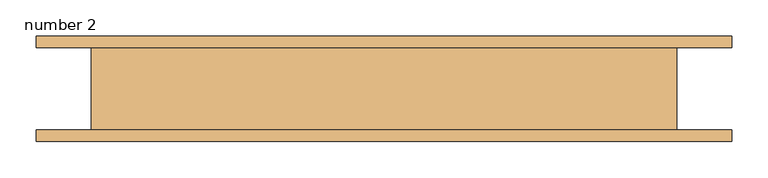
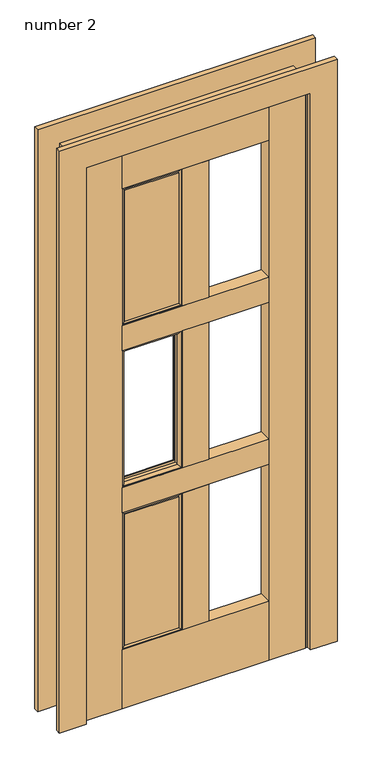
"""IFC4 building model written with IfcOpenShell, lengths in millimetres: door geometry, Door-Interior-Karona-K5660-6_Panel : number 2."""

from ifc_helpers import new_model, si_unit, frame, origin, origin_with_axes, place, context, project, spatial, polyline, ellipse_curve, outline, extrude, faceted_brep, source, transform, mapped, element, save
from ifc_brep_helpers import plane_surface, cylinder_surface, revolved_surface, advanced_brep


def number_2_d489d55d(model_context):
    return source(origin(), model_context, "Body", "SolidModel", [
        advanced_brep(
        [(-254.0, -15.2908, 1311.275), (-46.0375, -15.2908, 1311.275), (-57.3628137, -24.6126, 1299.9496863), (-242.6746863, -24.6126, 1299.9496863), (-57.1627, -46.3324899, 1300.1498), (-57.1627, -46.3324899, 820.7502), (-48.2727, -54.4576, 811.8602), (-48.2727, -54.4576, 1309.0398), (-242.8748, -46.3324899, 820.7502), (-242.8748, -46.3324899, 1300.1498), (-251.7648, -54.4576, 1309.0398), (-251.7648, -54.4576, 811.8602), (-46.0375, -54.4576, 809.625), (-254.0, -54.4576, 809.625), (-254.0, -15.2908, 809.625), (-46.0375, -15.2908, 809.625), (-57.1627, -34.7218, 820.7502), (-242.8748, -34.7218, 820.7502), (-47.3075, -24.6126, 1310.005), (-47.3075, -24.6126, 810.895), (-47.3075, -34.7218, 810.895), (-47.3075, -34.7218, 1310.005), (-252.73, -24.6126, 810.895), (-252.73, -24.6126, 1310.005), (-57.3628137, -24.6126, 820.9503137), (-242.6746863, -24.6126, 820.9503137), (-252.73, -34.7218, 810.895), (-254.0, -54.4576, 1311.275), (-242.8748, -34.7218, 1300.1498), (-252.73, -34.7218, 1310.005), (-46.0375, -54.4576, 1311.275), (-57.1627, -34.7218, 1300.1498)],
        [
            (0, 1),
            (1, 2, ellipse_curve(frame((-47.0685124, -25.5788135, 1310.2439876), z_axis=(-0.7071067811865475, 0.0, 0.7071067811865475), x_axis=(-0.7071067811865476, 0.0, -0.7071067811865474)), 14.6223259, 10.3395458)),
            (2, 3),
            (3, 0, ellipse_curve(frame((-252.9689876, -25.5788135, 1310.2439876), z_axis=(0.7071067811865475, 0.0, 0.7071067811865475), x_axis=(-0.7071067811865476, 0.0, 0.7071067811865474)), 14.6223259, 10.3395458)),
            (4, 5),
            (5, 6, ellipse_curve(frame((-48.2727, -45.531597, 811.8602), z_axis=(0.7071067811865475, 0.0, 0.7071067811865475), x_axis=(-0.7071067811865474, 0.0, 0.7071067811865476)), 12.6232745, 8.926003)),
            (6, 7),
            (7, 4, ellipse_curve(frame((-48.2727, -45.531597, 1309.0398), z_axis=(0.7071067811865475, 0.0, -0.7071067811865475), x_axis=(0.7071067811865474, 0.0, 0.7071067811865476)), 12.6232745, 8.926003)),
            (8, 9),
            (9, 10, ellipse_curve(frame((-251.7648, -45.531597, 1309.0398), z_axis=(-0.7071067811865475, 0.0, -0.7071067811865475), x_axis=(0.7071067811865474, 0.0, -0.7071067811865476)), 12.6232745, 8.926003)),
            (10, 11),
            (11, 8, ellipse_curve(frame((-251.7648, -45.531597, 811.8602), z_axis=(-0.7071067811865475, 0.0, 0.7071067811865475), x_axis=(-0.7071067811865474, 0.0, -0.7071067811865476)), 12.6232745, 8.926003)),
            (12, 13),
            (13, 14),
            (14, 15),
            (15, 12),
            (16, 17),
            (17, 8),
            (8, 5),
            (5, 16),
            (18, 19),
            (19, 20),
            (20, 21),
            (21, 18),
            (22, 19),
            (18, 23),
            (23, 22),
            (24, 25),
            (25, 3),
            (2, 24),
            (14, 25, ellipse_curve(frame((-252.9689876, -25.5788135, 810.6560124), z_axis=(0.7071067811865475, 0.0, -0.7071067811865475), x_axis=(0.7071067811865476, 0.0, 0.7071067811865474)), 14.6223259, 10.3395458)),
            (24, 15, ellipse_curve(frame((-47.0685124, -25.5788135, 810.6560124), z_axis=(-0.7071067811865475, 0.0, -0.7071067811865475), x_axis=(0.7071067811865476, 0.0, -0.7071067811865474)), 14.6223259, 10.3395458)),
            (22, 26),
            (26, 20),
            (13, 27),
            (27, 0),
            (0, 14),
            (17, 28),
            (28, 9),
            (23, 29),
            (29, 26),
            (27, 30),
            (30, 1),
            (28, 31),
            (31, 4),
            (4, 9),
            (21, 29),
            (30, 12),
            (15, 1),
            (31, 16),
            (6, 11),
            (10, 7),
        ],
        [
            cylinder_surface(frame((-254.0, -25.5788135, 1310.2439876), z_axis=(-1.0, 0.0, 0.0), x_axis=(0.0, 1.0, 0.0)), 10.3395458),
            cylinder_surface(frame((-48.2727, -45.531597, 1311.275), z_axis=(0.0, 0.0, 1.0), x_axis=(0.0, 1.0, 0.0)), 8.926003),
            cylinder_surface(frame((-251.7648, -45.531597, 809.625), z_axis=(0.0, 0.0, -1.0), x_axis=(0.0, 1.0, 0.0)), 8.926003),
            plane_surface(frame((-46.0375, -15.2908, 809.625), z_axis=(0.0, 0.0, -1.0), x_axis=(-1.0, 0.0, 0.0))),
            plane_surface(frame((-57.1627, -46.3324899, 820.7502), z_axis=(0.0, 0.0, 1.0), x_axis=(-1.0, 0.0, 0.0))),
            plane_surface(frame((-47.3075, -34.7218, 1310.005), z_axis=(-1.0, 0.0, 0.0), x_axis=(0.0, 0.0, -1.0))),
            plane_surface(frame((-47.3075, -24.6126, 1310.005), z_axis=(0.0, -1.0, 0.0), x_axis=(0.0, 0.0, -1.0))),
            cylinder_surface(frame((-46.0375, -25.5788135, 810.6560124), z_axis=(1.0, 0.0, 0.0), x_axis=(0.0, 1.0, 0.0)), 10.3395458),
            plane_surface(frame((-47.3075, -34.7218, 810.895), z_axis=(0.0, 0.0, 1.0), x_axis=(-1.0, 0.0, 0.0))),
            plane_surface(frame((-254.0, -15.2908, 809.625), z_axis=(-1.0, 0.0, 0.0), x_axis=(0.0, 0.0, 1.0))),
            plane_surface(frame((-242.8748, -46.3324899, 820.7502), z_axis=(1.0, 0.0, 0.0), x_axis=(0.0, 0.0, 1.0))),
            plane_surface(frame((-252.73, -34.7218, 810.895), z_axis=(1.0, 0.0, 0.0), x_axis=(0.0, 0.0, 1.0))),
            plane_surface(frame((-254.0, -15.2908, 1311.275), z_axis=(0.0, 0.0, 1.0), x_axis=(1.0, 0.0, 0.0))),
            plane_surface(frame((-242.8748, -46.3324899, 1300.1498), z_axis=(0.0, 0.0, -1.0), x_axis=(1.0, 0.0, 0.0))),
            plane_surface(frame((-252.73, -34.7218, 1310.005), z_axis=(0.0, 0.0, -1.0), x_axis=(1.0, 0.0, 0.0))),
            plane_surface(frame((-46.0375, -15.2908, 1311.275), z_axis=(1.0, 0.0, 0.0), x_axis=(0.0, 0.0, -1.0))),
            plane_surface(frame((-57.1627, -46.3324899, 1300.1498), z_axis=(-1.0, 0.0, 0.0), x_axis=(0.0, 0.0, -1.0))),
            plane_surface(frame((-57.1627, -34.7218, 1300.1498), z_axis=(0.0, 1.0, 0.0), x_axis=(0.0, 0.0, -1.0))),
            plane_surface(frame((-46.0375, -54.4576, 1311.275), z_axis=(0.0, -1.0, 0.0), x_axis=(0.0, 0.0, -1.0))),
            cylinder_surface(frame((-46.0375, -45.531597, 811.8602), z_axis=(1.0, 0.0, 0.0), x_axis=(0.0, 1.0, 0.0)), 8.926003),
            cylinder_surface(frame((-252.9689876, -25.5788135, 809.625), z_axis=(0.0, 0.0, -1.0), x_axis=(0.0, 1.0, 0.0)), 10.3395458),
            cylinder_surface(frame((-254.0, -45.531597, 1309.0398), z_axis=(-1.0, 0.0, 0.0), x_axis=(0.0, 1.0, 0.0)), 8.926003),
            cylinder_surface(frame((-47.0685124, -25.5788135, 1311.275), z_axis=(0.0, 0.0, 1.0), x_axis=(0.0, 1.0, 0.0)), 10.3395458),
        ],
        [
            (0, [[1, 2, 3, 4]]),
            (1, [[5, 6, 7, 8]]),
            (2, [[9, 10, 11, 12]]),
            (3, [[13, 14, 15, 16]]),
            (4, [[17, 18, 19, 20]]),
            (5, [[21, 22, 23, 24]]),
            (6, [[25, -21, 26, 27], [28, 29, -3, 30]]),
            (7, [[-15, 31, -28, 32]]),
            (8, [[-25, 33, 34, -22]]),
            (9, [[35, 36, 37, -14]]),
            (10, [[38, 39, -9, -18]]),
            (11, [[-27, 40, 41, -33]]),
            (12, [[42, 43, -1, -36]]),
            (13, [[44, 45, 46, -39]]),
            (14, [[-26, -24, 47, -40]]),
            (15, [[48, -16, 49, -43]]),
            (16, [[50, -20, -5, -45]]),
            (17, [[-34, -41, -47, -23], [-17, -50, -44, -38]]),
            (18, [[-13, -48, -42, -35], [51, -11, 52, -7]]),
            (19, [[-19, -12, -51, -6]]),
            (20, [[-37, -4, -29, -31]]),
            (21, [[-46, -8, -52, -10]]),
            (22, [[-49, -32, -30, -2]]),
        ],
    ),
        advanced_brep(
        [(-242.8748, -54.4576, 1893.8748), (-242.8748, -54.4576, 1414.4752), (-57.1627, -54.4576, 1414.4752), (-57.1627, -54.4576, 1893.8748), (-242.8748, -34.7218, 1893.8748), (-242.8748, -36.0454899, 1893.8748), (-57.1627, -36.0454899, 1893.8748), (-57.1627, -34.7218, 1893.8748), (-57.1627, -44.5515929, 1893.8748), (-242.8748, -44.5515929, 1893.8748), (-57.1627, -34.7218, 1414.4752), (-57.1627, -36.0454899, 1414.4752), (-242.8748, -36.0454899, 1414.4752), (-242.8748, -34.7218, 1414.4752), (-242.8748, -44.5515929, 1414.4752), (-57.1627, -44.5515929, 1414.4752), (-87.1686653, -44.5515929, 1863.8688347), (-212.8688347, -44.5515929, 1863.8688347), (-87.1686653, -44.5515929, 1444.4811653), (-212.8688347, -44.5515929, 1444.4811653)],
        [
            (0, 1),
            (1, 2),
            (2, 3),
            (3, 0),
            (4, 5),
            (5, 6),
            (6, 7),
            (7, 4),
            (3, 8),
            (8, 9),
            (9, 0),
            (10, 11),
            (11, 12),
            (12, 13),
            (13, 10),
            (1, 14),
            (14, 15),
            (15, 2),
            (9, 14),
            (12, 5),
            (4, 13),
            (6, 11),
            (10, 7),
            (15, 8),
            (16, 6, ellipse_curve(frame((-55.2243315, -100.0605261, 1895.8131685), z_axis=(0.7071067811865475, 0.0, -0.7071067811865475), x_axis=(-0.7071067811865476, 0.0, -0.7071067811865474)), 90.5724254, 64.0443762)),
            (5, 17, ellipse_curve(frame((-244.8131685, -100.0605261, 1895.8131685), z_axis=(-0.7071067811865475, 0.0, -0.7071067811865475), x_axis=(-0.7071067811865476, 0.0, 0.7071067811865474)), 90.5724254, 64.0443762)),
            (17, 16),
            (18, 11, ellipse_curve(frame((-55.2243315, -100.0605261, 1412.5368315), z_axis=(-0.7071067811865475, 0.0, -0.7071067811865475), x_axis=(-0.7071067811865474, 0.0, 0.7071067811865476)), 90.5724254, 64.0443762)),
            (16, 18),
            (19, 12, ellipse_curve(frame((-244.8131685, -100.0605261, 1412.5368315), z_axis=(-0.7071067811865475, 0.0, 0.7071067811865475), x_axis=(0.7071067811865476, 0.0, 0.7071067811865474)), 90.5724254, 64.0443762)),
            (18, 19),
            (19, 17),
        ],
        [
            plane_surface(frame((-57.1627, -54.4576, 1893.8748), z_axis=(0.0, -1.0, 0.0), x_axis=(0.0, 0.0, -1.0))),
            plane_surface(frame((-57.1627, -34.7218, 1893.8748), z_axis=(0.0, 0.0, 1.0), x_axis=(1.0, 0.0, 0.0))),
            plane_surface(frame((-57.1627, -34.7218, 1414.4752), z_axis=(0.0, 0.0, -1.0), x_axis=(-1.0, 0.0, 0.0))),
            plane_surface(frame((-242.8748, -54.4576, 1893.8748), z_axis=(-1.0, 0.0, 0.0), x_axis=(0.0, 0.0, -1.0))),
            plane_surface(frame((-57.1627, -34.7218, 1893.8748), z_axis=(1.0, 0.0, 0.0), x_axis=(0.0, 0.0, -1.0))),
            plane_surface(frame((-242.8748, -34.7218, 1893.8748), z_axis=(0.0, 1.0, 0.0), x_axis=(0.0, 0.0, -1.0))),
            revolved_surface(polyline([(-308.8575446888527, -100.0605261, 1831.7687923), (8.820044688852704, -100.0605261, 1831.7687923)]), (-254.0, -100.0605261, 1895.8131685), (-1.0, 0.0, 0.0)),
            revolved_surface(polyline([(-119.2687077, -100.0605261, 1959.8575446888528), (-119.2687077, -100.0605261, 1348.4924553111473)]), (-55.2243315, -100.0605261, 1905.0), (0.0, 0.0, 1.0)),
            revolved_surface(polyline([(8.820044688852683, -100.0605261, 1476.5812077), (-308.8575446888527, -100.0605261, 1476.5812077)]), (-46.0375, -100.0605261, 1412.5368315), (1.0, 0.0, 0.0)),
            revolved_surface(polyline([(-180.76879229999997, -100.0605261, 1348.4924553111473), (-180.76879229999997, -100.0605261, 1959.8575446888526)]), (-244.8131685, -100.0605261, 1403.35), (0.0, 0.0, -1.0)),
            plane_surface(frame((-254.0, -44.5515929, 1403.35), z_axis=(0.0, 1.0, 0.0), x_axis=(0.0, 0.0, 1.0))),
        ],
        [
            (0, [[1, 2, 3, 4]]),
            (1, [[5, 6, 7, 8]]),
            (1, [[9, 10, 11, -4]]),
            (2, [[12, 13, 14, 15]]),
            (2, [[16, 17, 18, -2]]),
            (3, [[-11, 19, -16, -1]]),
            (3, [[-14, 20, -5, 21]]),
            (4, [[-7, 22, -12, 23]]),
            (4, [[-18, 24, -9, -3]]),
            (5, [[-23, -15, -21, -8]]),
            (6, [[25, -6, 26, 27]]),
            (7, [[28, -22, -25, 29]]),
            (8, [[30, -13, -28, 31]]),
            (9, [[-26, -20, -30, 32]]),
            (10, [[-24, -17, -19, -10], [-32, -31, -29, -27]]),
        ],
    ),
        advanced_brep(
        [(-242.8748, -24.6126, 1893.8748), (-242.8748, -24.6126, 1414.4752), (-57.1627, -24.6126, 1414.4752), (-57.1627, -24.6126, 1893.8748), (-214.0448579, -15.4432, 1443.3051421), (-214.0448579, -15.4432, 1865.0448579), (-85.9926421, -15.4432, 1865.0448579), (-85.9926421, -15.4432, 1443.3051421), (-57.1627, -23.2889101, 1893.8748), (-242.8748, -23.2889101, 1893.8748), (-242.8748, -23.2889101, 1414.4752), (-57.1627, -23.2889101, 1414.4752)],
        [
            (0, 1),
            (1, 2),
            (2, 3),
            (3, 0),
            (4, 5),
            (5, 6),
            (6, 7),
            (7, 4),
            (3, 8),
            (8, 9),
            (9, 0),
            (1, 10),
            (10, 11),
            (11, 2),
            (7, 11, ellipse_curve(frame((-55.2243315, 40.7261261, 1412.5368315), z_axis=(0.7071067811865475, 0.0, 0.7071067811865475), x_axis=(0.7071067811865476, 0.0, -0.7071067811865474)), 90.5724254, 64.0443762)),
            (10, 4, ellipse_curve(frame((-244.8131685, 40.7261261, 1412.5368315), z_axis=(-0.7071067811865475, 0.0, 0.7071067811865475), x_axis=(0.7071067811865476, 0.0, 0.7071067811865474)), 90.5724254, 64.0443762)),
            (10, 9),
            (9, 5, ellipse_curve(frame((-244.8131685, 40.7261261, 1895.8131685), z_axis=(0.7071067811865475, 0.0, 0.7071067811865475), x_axis=(0.7071067811865474, 0.0, -0.7071067811865476)), 90.5724254, 64.0443762)),
            (8, 6, ellipse_curve(frame((-55.2243315, 40.7261261, 1895.8131685), z_axis=(0.7071067811865475, 0.0, -0.7071067811865475), x_axis=(-0.7071067811865476, 0.0, -0.7071067811865474)), 90.5724254, 64.0443762)),
            (8, 11),
        ],
        [
            plane_surface(frame((-57.1627, -24.6126, 1893.8748), z_axis=(0.0, -1.0, 0.0), x_axis=(0.0, 0.0, -1.0))),
            plane_surface(frame((-242.8748, -15.4432, 1893.8748), z_axis=(0.0, 1.0, 0.0), x_axis=(0.0, 0.0, -1.0))),
            plane_surface(frame((-57.1627, -34.7218, 1893.8748), z_axis=(0.0, 0.0, 1.0), x_axis=(1.0, 0.0, 0.0))),
            plane_surface(frame((-57.1627, -34.7218, 1414.4752), z_axis=(0.0, 0.0, -1.0), x_axis=(-1.0, 0.0, 0.0))),
            revolved_surface(polyline([(8.820044688852711, 40.7261261, 1476.5812077), (-308.8575446888527, 40.7261261, 1476.5812077)]), (-46.0375, 40.7261261, 1412.5368315), (1.0, 0.0, 0.0)),
            revolved_surface(polyline([(-180.76879229999997, 40.7261261, 1348.4924553111473), (-180.76879229999997, 40.7261261, 1959.8575446888528)]), (-244.8131685, 40.7261261, 1403.35), (0.0, 0.0, -1.0)),
            revolved_surface(polyline([(-308.85754468885267, 40.7261261, 1831.7687923), (8.820044688852704, 40.7261261, 1831.7687923)]), (-254.0, 40.7261261, 1895.8131685), (-1.0, 0.0, 0.0)),
            revolved_surface(polyline([(-119.2687077, 40.7261261, 1959.8575446888528), (-119.2687077, 40.7261261, 1348.4924553111473)]), (-55.2243315, 40.7261261, 1905.0), (0.0, 0.0, 1.0)),
            plane_surface(frame((-242.8748, -24.6126, 1893.8748), z_axis=(-1.0, 0.0, 0.0), x_axis=(0.0, 0.0, -1.0))),
            plane_surface(frame((-57.1627, -15.4432, 1893.8748), z_axis=(1.0, 0.0, 0.0), x_axis=(0.0, 0.0, -1.0))),
        ],
        [
            (0, [[1, 2, 3, 4]]),
            (1, [[5, 6, 7, 8]]),
            (2, [[9, 10, 11, -4]]),
            (3, [[12, 13, 14, -2]]),
            (4, [[-8, 15, -13, 16]]),
            (5, [[17, 18, -5, -16]]),
            (6, [[-10, 19, -6, -18]]),
            (7, [[20, -15, -7, -19]]),
            (8, [[-11, -17, -12, -1]]),
            (9, [[-14, -20, -9, -3]]),
        ],
    ),
        advanced_brep(
        [(-254.0, -15.2908, 1905.0), (-46.0375, -15.2908, 1905.0), (-57.3628137, -24.6126, 1893.6746863), (-242.6746863, -24.6126, 1893.6746863), (-57.1627, -46.3324899, 1893.8748), (-57.1627, -46.3324899, 1414.4752), (-48.2727, -54.4576, 1405.5852), (-48.2727, -54.4576, 1902.7648), (-242.8748, -46.3324899, 1414.4752), (-242.8748, -46.3324899, 1893.8748), (-251.7648, -54.4576, 1902.7648), (-251.7648, -54.4576, 1405.5852), (-46.0375, -54.4576, 1403.35), (-254.0, -54.4576, 1403.35), (-254.0, -15.2908, 1403.35), (-46.0375, -15.2908, 1403.35), (-57.1627, -34.7218, 1414.4752), (-242.8748, -34.7218, 1414.4752), (-47.3075, -24.6126, 1903.73), (-47.3075, -24.6126, 1404.62), (-47.3075, -34.7218, 1404.62), (-47.3075, -34.7218, 1903.73), (-252.73, -24.6126, 1404.62), (-252.73, -24.6126, 1903.73), (-57.3628137, -24.6126, 1414.6753137), (-242.6746863, -24.6126, 1414.6753137), (-252.73, -34.7218, 1404.62), (-254.0, -54.4576, 1905.0), (-242.8748, -34.7218, 1893.8748), (-252.73, -34.7218, 1903.73), (-46.0375, -54.4576, 1905.0), (-57.1627, -34.7218, 1893.8748)],
        [
            (0, 1),
            (1, 2, ellipse_curve(frame((-47.0685124, -25.5788135, 1903.9689876), z_axis=(-0.7071067811865475, 0.0, 0.7071067811865475), x_axis=(-0.7071067811865476, 0.0, -0.7071067811865474)), 14.6223259, 10.3395458)),
            (2, 3),
            (3, 0, ellipse_curve(frame((-252.9689876, -25.5788135, 1903.9689876), z_axis=(0.7071067811865475, 0.0, 0.7071067811865475), x_axis=(-0.7071067811865476, 0.0, 0.7071067811865474)), 14.6223259, 10.3395458)),
            (4, 5),
            (5, 6, ellipse_curve(frame((-48.2727, -45.531597, 1405.5852), z_axis=(0.7071067811865475, 0.0, 0.7071067811865475), x_axis=(-0.7071067811865474, 0.0, 0.7071067811865476)), 12.6232745, 8.926003)),
            (6, 7),
            (7, 4, ellipse_curve(frame((-48.2727, -45.531597, 1902.7648), z_axis=(0.7071067811865475, 0.0, -0.7071067811865475), x_axis=(0.7071067811865474, 0.0, 0.7071067811865476)), 12.6232745, 8.926003)),
            (8, 9),
            (9, 10, ellipse_curve(frame((-251.7648, -45.531597, 1902.7648), z_axis=(-0.7071067811865475, 0.0, -0.7071067811865475), x_axis=(0.7071067811865474, 0.0, -0.7071067811865476)), 12.6232745, 8.926003)),
            (10, 11),
            (11, 8, ellipse_curve(frame((-251.7648, -45.531597, 1405.5852), z_axis=(-0.7071067811865475, 0.0, 0.7071067811865475), x_axis=(-0.7071067811865474, 0.0, -0.7071067811865476)), 12.6232745, 8.926003)),
            (12, 13),
            (13, 14),
            (14, 15),
            (15, 12),
            (16, 17),
            (17, 8),
            (8, 5),
            (5, 16),
            (18, 19),
            (19, 20),
            (20, 21),
            (21, 18),
            (22, 19),
            (18, 23),
            (23, 22),
            (24, 25),
            (25, 3),
            (2, 24),
            (14, 25, ellipse_curve(frame((-252.9689876, -25.5788135, 1404.3810124), z_axis=(0.7071067811865475, 0.0, -0.7071067811865475), x_axis=(0.7071067811865476, 0.0, 0.7071067811865474)), 14.6223259, 10.3395458)),
            (24, 15, ellipse_curve(frame((-47.0685124, -25.5788135, 1404.3810124), z_axis=(-0.7071067811865475, 0.0, -0.7071067811865475), x_axis=(0.7071067811865476, 0.0, -0.7071067811865474)), 14.6223259, 10.3395458)),
            (22, 26),
            (26, 20),
            (13, 27),
            (27, 0),
            (0, 14),
            (17, 28),
            (28, 9),
            (23, 29),
            (29, 26),
            (27, 30),
            (30, 1),
            (28, 31),
            (31, 4),
            (4, 9),
            (21, 29),
            (30, 12),
            (15, 1),
            (31, 16),
            (6, 11),
            (10, 7),
        ],
        [
            cylinder_surface(frame((-254.0, -25.5788135, 1903.9689876), z_axis=(-1.0, 0.0, 0.0), x_axis=(0.0, 1.0, 0.0)), 10.3395458),
            cylinder_surface(frame((-48.2727, -45.531597, 1905.0), z_axis=(0.0, 0.0, 1.0), x_axis=(0.0, 1.0, 0.0)), 8.926003),
            cylinder_surface(frame((-251.7648, -45.531597, 1403.35), z_axis=(0.0, 0.0, -1.0), x_axis=(0.0, 1.0, 0.0)), 8.926003),
            plane_surface(frame((-46.0375, -15.2908, 1403.35), z_axis=(0.0, 0.0, -1.0), x_axis=(-1.0, 0.0, 0.0))),
            plane_surface(frame((-57.1627, -46.3324899, 1414.4752), z_axis=(0.0, 0.0, 1.0), x_axis=(-1.0, 0.0, 0.0))),
            plane_surface(frame((-47.3075, -34.7218, 1903.73), z_axis=(-1.0, 0.0, 0.0), x_axis=(0.0, 0.0, -1.0))),
            plane_surface(frame((-47.3075, -24.6126, 1903.73), z_axis=(0.0, -1.0, 0.0), x_axis=(0.0, 0.0, -1.0))),
            cylinder_surface(frame((-46.0375, -25.5788135, 1404.3810124), z_axis=(1.0, 0.0, 0.0), x_axis=(0.0, 1.0, 0.0)), 10.3395458),
            plane_surface(frame((-47.3075, -34.7218, 1404.62), z_axis=(0.0, 0.0, 1.0), x_axis=(-1.0, 0.0, 0.0))),
            plane_surface(frame((-254.0, -15.2908, 1403.35), z_axis=(-1.0, 0.0, 0.0), x_axis=(0.0, 0.0, 1.0))),
            plane_surface(frame((-242.8748, -46.3324899, 1414.4752), z_axis=(1.0, 0.0, 0.0), x_axis=(0.0, 0.0, 1.0))),
            plane_surface(frame((-252.73, -34.7218, 1404.62), z_axis=(1.0, 0.0, 0.0), x_axis=(0.0, 0.0, 1.0))),
            plane_surface(frame((-254.0, -15.2908, 1905.0), z_axis=(0.0, 0.0, 1.0), x_axis=(1.0, 0.0, 0.0))),
            plane_surface(frame((-242.8748, -46.3324899, 1893.8748), z_axis=(0.0, 0.0, -1.0), x_axis=(1.0, 0.0, 0.0))),
            plane_surface(frame((-252.73, -34.7218, 1903.73), z_axis=(0.0, 0.0, -1.0), x_axis=(1.0, 0.0, 0.0))),
            plane_surface(frame((-46.0375, -15.2908, 1905.0), z_axis=(1.0, 0.0, 0.0), x_axis=(0.0, 0.0, -1.0))),
            plane_surface(frame((-57.1627, -46.3324899, 1893.8748), z_axis=(-1.0, 0.0, 0.0), x_axis=(0.0, 0.0, -1.0))),
            plane_surface(frame((-57.1627, -34.7218, 1893.8748), z_axis=(0.0, 1.0, 0.0), x_axis=(0.0, 0.0, -1.0))),
            plane_surface(frame((-46.0375, -54.4576, 1905.0), z_axis=(0.0, -1.0, 0.0), x_axis=(0.0, 0.0, -1.0))),
            cylinder_surface(frame((-46.0375, -45.531597, 1405.5852), z_axis=(1.0, 0.0, 0.0), x_axis=(0.0, 1.0, 0.0)), 8.926003),
            cylinder_surface(frame((-252.9689876, -25.5788135, 1403.35), z_axis=(0.0, 0.0, -1.0), x_axis=(0.0, 1.0, 0.0)), 10.3395458),
            cylinder_surface(frame((-254.0, -45.531597, 1902.7648), z_axis=(-1.0, 0.0, 0.0), x_axis=(0.0, 1.0, 0.0)), 8.926003),
            cylinder_surface(frame((-47.0685124, -25.5788135, 1905.0), z_axis=(0.0, 0.0, 1.0), x_axis=(0.0, 1.0, 0.0)), 10.3395458),
        ],
        [
            (0, [[1, 2, 3, 4]]),
            (1, [[5, 6, 7, 8]]),
            (2, [[9, 10, 11, 12]]),
            (3, [[13, 14, 15, 16]]),
            (4, [[17, 18, 19, 20]]),
            (5, [[21, 22, 23, 24]]),
            (6, [[25, -21, 26, 27], [28, 29, -3, 30]]),
            (7, [[-15, 31, -28, 32]]),
            (8, [[-25, 33, 34, -22]]),
            (9, [[35, 36, 37, -14]]),
            (10, [[38, 39, -9, -18]]),
            (11, [[-27, 40, 41, -33]]),
            (12, [[42, 43, -1, -36]]),
            (13, [[44, 45, 46, -39]]),
            (14, [[-26, -24, 47, -40]]),
            (15, [[48, -16, 49, -43]]),
            (16, [[50, -20, -5, -45]]),
            (17, [[-34, -41, -47, -23], [-17, -50, -44, -38]]),
            (18, [[-13, -48, -42, -35], [51, -11, 52, -7]]),
            (19, [[-19, -12, -51, -6]]),
            (20, [[-37, -4, -29, -31]]),
            (21, [[-46, -8, -52, -10]]),
            (22, [[-49, -32, -30, -2]]),
        ],
    ),
        advanced_brep(
        [(-242.8748, -34.7218, 706.4248), (-242.8748, -36.0454899, 706.4248), (-57.1627, -36.0454899, 706.4248), (-57.1627, -34.7218, 706.4248), (-57.1627, -54.4576, 706.4248), (-57.1627, -44.5515929, 706.4248), (-242.8748, -44.5515929, 706.4248), (-242.8748, -54.4576, 706.4248), (-57.1627, -34.7218, 227.0252), (-57.1627, -36.0454899, 227.0252), (-242.8748, -36.0454899, 227.0252), (-242.8748, -34.7218, 227.0252), (-242.8748, -54.4576, 227.0252), (-242.8748, -44.5515929, 227.0252), (-57.1627, -44.5515929, 227.0252), (-57.1627, -54.4576, 227.0252), (-87.1686653, -44.5515929, 676.4188347), (-212.8688347, -44.5515929, 676.4188347), (-87.1686653, -44.5515929, 257.0311653), (-212.8688347, -44.5515929, 257.0311653)],
        [
            (0, 1),
            (1, 2),
            (2, 3),
            (3, 0),
            (4, 5),
            (5, 6),
            (6, 7),
            (7, 4),
            (8, 9),
            (9, 10),
            (10, 11),
            (11, 8),
            (12, 13),
            (13, 14),
            (14, 15),
            (15, 12),
            (6, 13),
            (12, 7),
            (10, 1),
            (0, 11),
            (15, 4),
            (2, 9),
            (8, 3),
            (14, 5),
            (16, 2, ellipse_curve(frame((-55.2243315, -100.0605261, 708.3631685), z_axis=(0.7071067811865475, 0.0, -0.7071067811865475), x_axis=(-0.7071067811865476, 0.0, -0.7071067811865474)), 90.5724254, 64.0443762)),
            (1, 17, ellipse_curve(frame((-244.8131685, -100.0605261, 708.3631685), z_axis=(-0.7071067811865475, 0.0, -0.7071067811865475), x_axis=(-0.7071067811865476, 0.0, 0.7071067811865474)), 90.5724254, 64.0443762)),
            (17, 16),
            (18, 9, ellipse_curve(frame((-55.2243315, -100.0605261, 225.0868315), z_axis=(-0.7071067811865475, 0.0, -0.7071067811865475), x_axis=(-0.7071067811865474, 0.0, 0.7071067811865476)), 90.5724254, 64.0443762)),
            (16, 18),
            (19, 10, ellipse_curve(frame((-244.8131685, -100.0605261, 225.0868315), z_axis=(-0.7071067811865475, 0.0, 0.7071067811865475), x_axis=(0.7071067811865476, 0.0, 0.7071067811865474)), 90.5724254, 64.0443762)),
            (18, 19),
            (19, 17),
        ],
        [
            plane_surface(frame((-57.1627, -34.7218, 706.4248), z_axis=(0.0, 0.0, 1.0), x_axis=(1.0, 0.0, 0.0))),
            plane_surface(frame((-57.1627, -34.7218, 227.0252), z_axis=(0.0, 0.0, -1.0), x_axis=(-1.0, 0.0, 0.0))),
            plane_surface(frame((-242.8748, -54.4576, 706.4248), z_axis=(-1.0, 0.0, 0.0), x_axis=(0.0, 0.0, -1.0))),
            plane_surface(frame((-57.1627, -54.4576, 706.4248), z_axis=(0.0, -1.0, 0.0), x_axis=(0.0, 0.0, -1.0))),
            plane_surface(frame((-57.1627, -34.7218, 706.4248), z_axis=(1.0, 0.0, 0.0), x_axis=(0.0, 0.0, -1.0))),
            plane_surface(frame((-242.8748, -34.7218, 706.4248), z_axis=(0.0, 1.0, 0.0), x_axis=(0.0, 0.0, -1.0))),
            revolved_surface(polyline([(-308.8575446888527, -100.0605261, 644.3187923), (8.820044688852704, -100.0605261, 644.3187923)]), (-254.0, -100.0605261, 708.3631685), (-1.0, 0.0, 0.0)),
            revolved_surface(polyline([(-119.2687077, -100.0605261, 772.4075446888527), (-119.2687077, -100.0605261, 161.04245531114725)]), (-55.2243315, -100.0605261, 717.55), (0.0, 0.0, 1.0)),
            revolved_surface(polyline([(8.820044688852683, -100.0605261, 289.1312077), (-308.8575446888527, -100.0605261, 289.1312077)]), (-46.0375, -100.0605261, 225.0868315), (1.0, 0.0, 0.0)),
            revolved_surface(polyline([(-180.76879229999997, -100.0605261, 161.0424553111473), (-180.76879229999997, -100.0605261, 772.4075446888527)]), (-244.8131685, -100.0605261, 215.9), (0.0, 0.0, -1.0)),
            plane_surface(frame((-254.0, -44.5515929, 215.9), z_axis=(0.0, 1.0, 0.0), x_axis=(0.0, 0.0, 1.0))),
        ],
        [
            (0, [[1, 2, 3, 4]]),
            (0, [[5, 6, 7, 8]]),
            (1, [[9, 10, 11, 12]]),
            (1, [[13, 14, 15, 16]]),
            (2, [[-7, 17, -13, 18]]),
            (2, [[-11, 19, -1, 20]]),
            (3, [[-18, -16, 21, -8]]),
            (4, [[-3, 22, -9, 23]]),
            (4, [[-15, 24, -5, -21]]),
            (5, [[-23, -12, -20, -4]]),
            (6, [[25, -2, 26, 27]]),
            (7, [[28, -22, -25, 29]]),
            (8, [[30, -10, -28, 31]]),
            (9, [[-26, -19, -30, 32]]),
            (10, [[-24, -14, -17, -6], [-32, -31, -29, -27]]),
        ],
    ),
        advanced_brep(
        [(-57.1627, -24.6126, 706.4248), (-57.1627, -23.2889101, 706.4248), (-242.8748, -23.2889101, 706.4248), (-242.8748, -24.6126, 706.4248), (-242.8748, -24.6126, 227.0252), (-242.8748, -23.2889101, 227.0252), (-57.1627, -23.2889101, 227.0252), (-57.1627, -24.6126, 227.0252), (-214.0448579, -15.4432, 255.8551421), (-214.0448579, -15.4432, 677.5948579), (-85.9926421, -15.4432, 677.5948579), (-85.9926421, -15.4432, 255.8551421)],
        [
            (0, 1),
            (1, 2),
            (2, 3),
            (3, 0),
            (4, 5),
            (5, 6),
            (6, 7),
            (7, 4),
            (3, 4),
            (7, 0),
            (8, 9),
            (9, 10),
            (10, 11),
            (11, 8),
            (11, 6, ellipse_curve(frame((-55.2243315, 40.7261261, 225.0868315), z_axis=(0.7071067811865475, 0.0, 0.7071067811865475), x_axis=(0.7071067811865476, 0.0, -0.7071067811865474)), 90.5724254, 64.0443762)),
            (5, 8, ellipse_curve(frame((-244.8131685, 40.7261261, 225.0868315), z_axis=(-0.7071067811865475, 0.0, 0.7071067811865475), x_axis=(0.7071067811865476, 0.0, 0.7071067811865474)), 90.5724254, 64.0443762)),
            (5, 2),
            (2, 9, ellipse_curve(frame((-244.8131685, 40.7261261, 708.3631685), z_axis=(0.7071067811865475, 0.0, 0.7071067811865475), x_axis=(0.7071067811865474, 0.0, -0.7071067811865476)), 90.5724254, 64.0443762)),
            (1, 10, ellipse_curve(frame((-55.2243315, 40.7261261, 708.3631685), z_axis=(0.7071067811865475, 0.0, -0.7071067811865475), x_axis=(-0.7071067811865476, 0.0, -0.7071067811865474)), 90.5724254, 64.0443762)),
            (1, 6),
        ],
        [
            plane_surface(frame((-57.1627, -34.7218, 706.4248), z_axis=(0.0, 0.0, 1.0), x_axis=(1.0, 0.0, 0.0))),
            plane_surface(frame((-57.1627, -34.7218, 227.0252), z_axis=(0.0, 0.0, -1.0), x_axis=(-1.0, 0.0, 0.0))),
            plane_surface(frame((-57.1627, -24.6126, 706.4248), z_axis=(0.0, -1.0, 0.0), x_axis=(0.0, 0.0, -1.0))),
            plane_surface(frame((-242.8748, -15.4432, 706.4248), z_axis=(0.0, 1.0, 0.0), x_axis=(0.0, 0.0, -1.0))),
            revolved_surface(polyline([(8.820044688852711, 40.7261261, 289.1312077), (-308.8575446888527, 40.7261261, 289.1312077)]), (-46.0375, 40.7261261, 225.0868315), (1.0, 0.0, 0.0)),
            revolved_surface(polyline([(-180.76879229999997, 40.7261261, 161.0424553111473), (-180.76879229999997, 40.7261261, 772.4075446888527)]), (-244.8131685, 40.7261261, 215.9), (0.0, 0.0, -1.0)),
            revolved_surface(polyline([(-308.85754468885267, 40.7261261, 644.3187923), (8.820044688852704, 40.7261261, 644.3187923)]), (-254.0, 40.7261261, 708.3631685), (-1.0, 0.0, 0.0)),
            revolved_surface(polyline([(-119.2687077, 40.7261261, 772.4075446888527), (-119.2687077, 40.7261261, 161.04245531114736)]), (-55.2243315, 40.7261261, 717.55), (0.0, 0.0, 1.0)),
            plane_surface(frame((-242.8748, -24.6126, 706.4248), z_axis=(-1.0, 0.0, 0.0), x_axis=(0.0, 0.0, -1.0))),
            plane_surface(frame((-57.1627, -15.4432, 706.4248), z_axis=(1.0, 0.0, 0.0), x_axis=(0.0, 0.0, -1.0))),
        ],
        [
            (0, [[1, 2, 3, 4]]),
            (1, [[5, 6, 7, 8]]),
            (2, [[9, -8, 10, -4]]),
            (3, [[11, 12, 13, 14]]),
            (4, [[-14, 15, -6, 16]]),
            (5, [[17, 18, -11, -16]]),
            (6, [[-2, 19, -12, -18]]),
            (7, [[20, -15, -13, -19]]),
            (8, [[-3, -17, -5, -9]]),
            (9, [[-7, -20, -1, -10]]),
        ],
    ),
        advanced_brep(
        [(-254.0, -15.2908, 717.55), (-46.0375, -15.2908, 717.55), (-57.3628137, -24.6126, 706.2246863), (-242.6746863, -24.6126, 706.2246863), (-57.1627, -46.3324899, 706.4248), (-57.1627, -46.3324899, 227.0252), (-48.2727, -54.4576, 218.1352), (-48.2727, -54.4576, 715.3148), (-254.0, -54.4576, 215.9), (-46.0375, -54.4576, 215.9), (-46.0375, -54.4576, 717.55), (-254.0, -54.4576, 717.55), (-251.7648, -54.4576, 218.1352), (-251.7648, -54.4576, 715.3148), (-254.0, -15.2908, 215.9), (-46.0375, -15.2908, 215.9), (-57.1627, -34.7218, 227.0252), (-242.8748, -34.7218, 227.0252), (-242.8748, -46.3324899, 227.0252), (-47.3075, -24.6126, 217.17), (-252.73, -24.6126, 217.17), (-252.73, -34.7218, 217.17), (-47.3075, -34.7218, 217.17), (-242.8748, -34.7218, 706.4248), (-242.8748, -46.3324899, 706.4248), (-252.73, -24.6126, 716.28), (-252.73, -34.7218, 716.28), (-57.1627, -34.7218, 706.4248), (-47.3075, -24.6126, 716.28), (-47.3075, -34.7218, 716.28), (-57.3628137, -24.6126, 227.2253137), (-242.6746863, -24.6126, 227.2253137)],
        [
            (0, 1),
            (1, 2, ellipse_curve(frame((-47.0685124, -25.5788135, 716.5189876), z_axis=(-0.7071067811865475, 0.0, 0.7071067811865475), x_axis=(-0.7071067811865476, 0.0, -0.7071067811865474)), 14.6223259, 10.3395458)),
            (2, 3),
            (3, 0, ellipse_curve(frame((-252.9689876, -25.5788135, 716.5189876), z_axis=(0.7071067811865475, 0.0, 0.7071067811865475), x_axis=(-0.7071067811865476, 0.0, 0.7071067811865474)), 14.6223259, 10.3395458)),
            (4, 5),
            (5, 6, ellipse_curve(frame((-48.2727, -45.531597, 218.1352), z_axis=(0.7071067811865475, 0.0, 0.7071067811865475), x_axis=(-0.7071067811865474, 0.0, 0.7071067811865476)), 12.6232745, 8.926003)),
            (6, 7),
            (7, 4, ellipse_curve(frame((-48.2727, -45.531597, 715.3148), z_axis=(0.7071067811865475, 0.0, -0.7071067811865475), x_axis=(0.7071067811865474, 0.0, 0.7071067811865476)), 12.6232745, 8.926003)),
            (8, 9),
            (9, 10),
            (10, 11),
            (11, 8),
            (6, 12),
            (12, 13),
            (13, 7),
            (8, 14),
            (14, 15),
            (15, 9),
            (16, 17),
            (17, 18),
            (18, 5),
            (5, 16),
            (19, 20),
            (20, 21),
            (21, 22),
            (22, 19),
            (11, 0),
            (0, 14),
            (17, 23),
            (23, 24),
            (24, 18),
            (20, 25),
            (25, 26),
            (26, 21),
            (10, 1),
            (23, 27),
            (27, 4),
            (4, 24),
            (25, 28),
            (28, 29),
            (29, 26),
            (15, 1),
            (27, 16),
            (29, 22),
            (28, 19),
            (30, 31),
            (31, 3),
            (2, 30),
            (15, 30, ellipse_curve(frame((-47.0685124, -25.5788135, 216.9310124), z_axis=(0.7071067811865475, 0.0, 0.7071067811865475), x_axis=(-0.7071067811865474, 0.0, 0.7071067811865476)), 14.6223259, 10.3395458)),
            (24, 13, ellipse_curve(frame((-251.7648, -45.531597, 715.3148), z_axis=(-0.7071067811865475, 0.0, -0.7071067811865475), x_axis=(0.7071067811865474, 0.0, -0.7071067811865476)), 12.6232745, 8.926003)),
            (12, 18, ellipse_curve(frame((-251.7648, -45.531597, 218.1352), z_axis=(-0.7071067811865475, 0.0, 0.7071067811865475), x_axis=(-0.7071067811865474, 0.0, -0.7071067811865476)), 12.6232745, 8.926003)),
            (14, 31, ellipse_curve(frame((-252.9689876, -25.5788135, 216.9310124), z_axis=(0.7071067811865475, 0.0, -0.7071067811865475), x_axis=(0.7071067811865476, 0.0, 0.7071067811865474)), 14.6223259, 10.3395458)),
        ],
        [
            cylinder_surface(frame((-254.0, -25.5788135, 716.5189876), z_axis=(-1.0, 0.0, 0.0), x_axis=(0.0, 1.0, 0.0)), 10.3395458),
            cylinder_surface(frame((-48.2727, -45.531597, 717.55), z_axis=(0.0, 0.0, 1.0), x_axis=(0.0, 1.0, 0.0)), 8.926003),
            plane_surface(frame((-46.0375, -54.4576, 717.55), z_axis=(0.0, -1.0, 0.0), x_axis=(0.0, 0.0, -1.0))),
            plane_surface(frame((-46.0375, -15.2908, 215.9), z_axis=(0.0, 0.0, -1.0), x_axis=(-1.0, 0.0, 0.0))),
            plane_surface(frame((-57.1627, -46.3324899, 227.0252), z_axis=(0.0, 0.0, 1.0), x_axis=(-1.0, 0.0, 0.0))),
            plane_surface(frame((-47.3075, -34.7218, 217.17), z_axis=(0.0, 0.0, 1.0), x_axis=(-1.0, 0.0, 0.0))),
            plane_surface(frame((-254.0, -15.2908, 215.9), z_axis=(-1.0, 0.0, 0.0), x_axis=(0.0, 0.0, 1.0))),
            plane_surface(frame((-242.8748, -46.3324899, 227.0252), z_axis=(1.0, 0.0, 0.0), x_axis=(0.0, 0.0, 1.0))),
            plane_surface(frame((-252.73, -34.7218, 217.17), z_axis=(1.0, 0.0, 0.0), x_axis=(0.0, 0.0, 1.0))),
            plane_surface(frame((-254.0, -15.2908, 717.55), z_axis=(0.0, 0.0, 1.0), x_axis=(1.0, 0.0, 0.0))),
            plane_surface(frame((-242.8748, -46.3324899, 706.4248), z_axis=(0.0, 0.0, -1.0), x_axis=(1.0, 0.0, 0.0))),
            plane_surface(frame((-252.73, -34.7218, 716.28), z_axis=(0.0, 0.0, -1.0), x_axis=(1.0, 0.0, 0.0))),
            plane_surface(frame((-46.0375, -15.2908, 717.55), z_axis=(1.0, 0.0, 0.0), x_axis=(0.0, 0.0, -1.0))),
            plane_surface(frame((-57.1627, -46.3324899, 706.4248), z_axis=(-1.0, 0.0, 0.0), x_axis=(0.0, 0.0, -1.0))),
            plane_surface(frame((-57.1627, -34.7218, 706.4248), z_axis=(0.0, 1.0, 0.0), x_axis=(0.0, 0.0, -1.0))),
            plane_surface(frame((-47.3075, -34.7218, 716.28), z_axis=(-1.0, 0.0, 0.0), x_axis=(0.0, 0.0, -1.0))),
            plane_surface(frame((-47.3075, -24.6126, 716.28), z_axis=(0.0, -1.0, 0.0), x_axis=(0.0, 0.0, -1.0))),
            cylinder_surface(frame((-47.0685124, -25.5788135, 717.55), z_axis=(0.0, 0.0, 1.0), x_axis=(0.0, 1.0, 0.0)), 10.3395458),
            cylinder_surface(frame((-251.7648, -45.531597, 215.9), z_axis=(0.0, 0.0, -1.0), x_axis=(0.0, 1.0, 0.0)), 8.926003),
            cylinder_surface(frame((-46.0375, -25.5788135, 216.9310124), z_axis=(1.0, 0.0, 0.0), x_axis=(0.0, 1.0, 0.0)), 10.3395458),
            cylinder_surface(frame((-46.0375, -45.531597, 218.1352), z_axis=(1.0, 0.0, 0.0), x_axis=(0.0, 1.0, 0.0)), 8.926003),
            cylinder_surface(frame((-252.9689876, -25.5788135, 215.9), z_axis=(0.0, 0.0, -1.0), x_axis=(0.0, 1.0, 0.0)), 10.3395458),
            cylinder_surface(frame((-254.0, -45.531597, 715.3148), z_axis=(-1.0, 0.0, 0.0), x_axis=(0.0, 1.0, 0.0)), 8.926003),
        ],
        [
            (0, [[1, 2, 3, 4]]),
            (1, [[5, 6, 7, 8]]),
            (2, [[9, 10, 11, 12], [13, 14, 15, -7]]),
            (3, [[-9, 16, 17, 18]]),
            (4, [[19, 20, 21, 22]]),
            (5, [[23, 24, 25, 26]]),
            (6, [[-12, 27, 28, -16]]),
            (7, [[29, 30, 31, -20]]),
            (8, [[32, 33, 34, -24]]),
            (9, [[-11, 35, -1, -27]]),
            (10, [[36, 37, 38, -30]]),
            (11, [[39, 40, 41, -33]]),
            (12, [[-10, -18, 42, -35]]),
            (13, [[43, -22, -5, -37]]),
            (14, [[-25, -34, -41, 44], [-19, -43, -36, -29]]),
            (15, [[45, -26, -44, -40]]),
            (16, [[-23, -45, -39, -32], [46, 47, -3, 48]]),
            (17, [[-42, 49, -48, -2]]),
            (18, [[-31, 50, -14, 51]]),
            (19, [[-17, 52, -46, -49]]),
            (20, [[-21, -51, -13, -6]]),
            (21, [[-28, -4, -47, -52]]),
            (22, [[-38, -8, -15, -50]]),
        ],
    ),
        extrude(outline(polyline([(254.0, -12.7), (254.0, -57.15), (-254.0, -57.15), (-254.0, -12.7), (254.0, -12.7)])), frame((0.0, 0.0, 1905.0), z_axis=(0.0, 0.0, 1.0), x_axis=(1.0, 0.0, 0.0)), (0.0, 0.0, 1.0), 127.0),
        extrude(outline(polyline([(254.0, -12.7), (254.0, -57.15), (-254.0, -57.15), (-254.0, -12.7), (254.0, -12.7)])), origin_with_axes(), (0.0, 0.0, 1.0), 215.9),
        extrude(outline(polyline([(46.0375, -12.7), (46.0375, -57.15), (-46.0375, -57.15), (-46.0375, -12.7), (46.0375, -12.7)])), frame((0.0, 0.0, 215.9), z_axis=(0.0, 0.0, 1.0), x_axis=(1.0, 0.0, 0.0)), (0.0, 0.0, 1.0), 501.65),
        extrude(outline(polyline([(46.0375, -12.7), (46.0375, -57.15), (-46.0375, -57.15), (-46.0375, -12.7), (46.0375, -12.7)])), frame((0.0, 0.0, 809.625), z_axis=(0.0, 0.0, 1.0), x_axis=(1.0, 0.0, 0.0)), (0.0, 0.0, 1.0), 501.65),
        extrude(outline(polyline([(46.0375, -12.7), (46.0375, -57.15), (-46.0375, -57.15), (-46.0375, -12.7), (46.0375, -12.7)])), frame((0.0, 0.0, 1403.35), z_axis=(0.0, 0.0, 1.0), x_axis=(1.0, 0.0, 0.0)), (0.0, 0.0, 1.0), 501.65),
        extrude(outline(polyline([(254.0, -12.7), (254.0, -57.15), (-254.0, -57.15), (-254.0, -12.7), (254.0, -12.7)])), frame((0.0, 0.0, 717.55), z_axis=(0.0, 0.0, 1.0), x_axis=(1.0, 0.0, 0.0)), (0.0, 0.0, 1.0), 92.075),
        extrude(outline(polyline([(254.0, -12.7), (254.0, -57.15), (-254.0, -57.15), (-254.0, -12.7), (254.0, -12.7)])), frame((0.0, 0.0, 1311.275), z_axis=(0.0, 0.0, 1.0), x_axis=(1.0, 0.0, 0.0)), (0.0, 0.0, 1.0), 92.075),
        extrude(outline(polyline([(381.0, -12.7), (381.0, -57.15), (254.0, -57.15), (254.0, -12.7), (381.0, -12.7)])), origin_with_axes(), (0.0, 0.0, 1.0), 2032.0),
        extrude(outline(polyline([(-254.0, -12.7), (-254.0, -57.15), (-381.0, -57.15), (-381.0, -12.7), (-254.0, -12.7)])), origin_with_axes(), (0.0, 0.0, 1.0), 2032.0),
        faceted_brep([(405.209375, 57.15, 0.0), (405.209375, -57.15, 0.0), (382.190625, -57.15, 0.0), (382.190625, -12.7, 0.0), (367.4401275, -12.7, 0.0), (367.4401275, 22.225, 0.0), (382.190625, 22.225, 0.0), (382.190625, 57.15, 0.0), (382.190625, 57.15, 2033.190625), (-382.190625, 57.15, 2033.190625), (-382.190625, 57.15, 0.0), (-405.209375, 57.15, 0.0), (-405.209375, 57.15, 2056.209375), (405.209375, 57.15, 2056.209375), (382.190625, 22.225, 2033.190625), (367.4401275, 22.225, 2018.4401275), (-367.4401275, 22.225, 2018.4401275), (-367.4401275, 22.225, 0.0), (-382.190625, 22.225, 0.0), (-382.190625, 22.225, 2033.190625), (367.4401275, -12.7, 2018.4401275), (382.190625, -12.7, 2033.190625), (-382.190625, -12.7, 2033.190625), (-382.190625, -12.7, 0.0), (-367.4401275, -12.7, 0.0), (-367.4401275, -12.7, 2018.4401275), (382.190625, -57.15, 2033.190625), (405.209375, -57.15, 2056.209375), (-405.209375, -57.15, 2056.209375), (-405.209375, -57.15, 0.0), (-382.190625, -57.15, 0.0), (-382.190625, -57.15, 2033.190625)], [[[0, 1, 2, 3, 4, 5, 6, 7]], [[7, 8, 9, 10, 11, 12, 13, 0]], [[6, 14, 8, 7]], [[5, 15, 16, 17, 18, 19, 14, 6]], [[4, 20, 15, 5]], [[3, 21, 22, 23, 24, 25, 20, 4]], [[2, 26, 21, 3]], [[1, 27, 28, 29, 30, 31, 26, 2]], [[0, 13, 27, 1]], [[14, 19, 9, 8]], [[20, 25, 16, 15]], [[26, 31, 22, 21]], [[13, 12, 28, 27]], [[11, 10, 18, 17, 24, 23, 30, 29]], [[19, 18, 10, 9]], [[25, 24, 17, 16]], [[31, 30, 23, 22]], [[12, 11, 29, 28]]]),
        extrude(outline(polyline([(2132.409375, -481.409375), (0.0, -481.409375), (0.0, -388.540625), (2039.540625, -388.540625), (2039.540625, 388.540625), (0.0, 388.540625), (0.0, 481.409375), (2132.409375, 481.409375), (2132.409375, -481.409375)])), frame((0.0, 57.15, 0.0), z_axis=(0.0, 1.0, 0.0), x_axis=(0.0, 0.0, 1.0)), (0.0, 0.0, 1.0), 15.875),
        extrude(outline(polyline([(2132.409375, 481.409375), (2132.409375, -481.409375), (0.0, -481.409375), (0.0, -388.540625), (2039.540625, -388.540625), (2039.540625, 388.540625), (0.0, 388.540625), (0.0, 481.409375), (2132.409375, 481.409375)])), frame((0.0, -73.025, 0.0), z_axis=(0.0, 1.0, 0.0), x_axis=(0.0, 0.0, 1.0)), (0.0, 0.0, 1.0), 15.875),
    ])


if __name__ == "__main__":
    model = new_model("IFC4")
    model_context = context("Model", 3, world=origin())
    ifc_project = project(units=[si_unit("LENGTHUNIT", "METRE", prefix="MILLI")], contexts=[model_context])
    site = spatial("IfcSite", under=ifc_project)
    building = spatial("IfcBuilding", under=site)
    placement = place(None, origin())
    number_2_shape = number_2_d489d55d(model_context)
    element("IfcDoor", 1, ObjectType="Door-Interior-Karona-K5660-6_Panel : number 2", at=placement, inside=building, context=model_context, shape_type="MappedRepresentation", body=[
        mapped(number_2_shape, transform((0.0, 0.0, 0.0), x_axis=(1.0, 0.0, 0.0), y_axis=(0.0, 1.0, 0.0), z_axis=(0.0, 0.0, 1.0))),
    ])
    save(model, "model.ifc")

# Revit data of these elements
# Type "Door-Interior-Karona-K5660-6_Panel : number 2"
#   Type Mark = "82"
#   Youtube clip = ""
#   Warranty URL = "http://www.karonadoor.com/pdf/literature/Warranty_.pdf"
#   Warranty = "Limited lifetime warranty on all interior doors."
#   Uniformat II Description = ""
#   Uniformat II Code = ""
#   Uniclass 2015 Name = "Doorsets"
#   Uniclass 2015 Code = "Pr_30_59_24"
#   Uniclass 2.0 Description = "Doorsets"
#   Uniclass 2.0 Code = "PR-59-23"
#   Uniclass 1.4 Description = "Doors"
#   Uniclass 1.4 Code = "JL20"
#   URL = "http://www.karonadoor.com/"
#   UNSPSC Code = "30171511"
#   Technical description = "http://www.karonadoor.com/pdf/Architectural.Guide.pdf"
#   Support Email = "mailto:bimsupport@jeldwen.com"
#   Region South America = "None"
#   Region Oceania = "None"
#   Region North America = "CA, US"
#   Region Middle East = "None"
#   Region Europe = "None"
#   Region Asia = "None"
#   Region Antarctica = "None"
#   Region Africa = "None"
#   QR code = "http://bimobject.com/karona/product/K5660"
#   Product url = "http://www.karonadoor.com/commercial_products.php?category_id=1&style_id=1&image_id=21"
#   Product group = "Panel Doors"
#   Product family = "Commercial Products"
#   Product data url = "https://bimobject.com/karona/product/K5660"
#   Product certification = ""
#   Product SKU = "K5660"
#   Product Guid = "0ef6a8f4-4242-4391-b579-45df545b9ddd"
#   Operation = "Swing"
#   OmniClass Description = "Wood Doors"
#   OmniClass Code = "23-17 11 15"
#   NBS Reference Description = "Doorsets"
#   NBS Reference Code = "59-23"
#   Model = "K5660"
#   Material secondary = ""
#   Material main = "Wood"
#   Masterformat 2014 Description = "Stile and Rail Wood Doors"
#   Masterformat 2014 Code = "08 14 33"
#   Manufacturer name = "Karona"
#   Manufacturer country = "United States"
#   Manufacturer = "Karona Door, Inc."
#   Keynote = "08 14 33"
#   Installation instructions = ""
#   IFC Classification = "Door"
#   Green Product Information = "Available in Certified Wood, No-added Urea, & Recycled"
#   Fire Rating Data = "http://www.karonadoor.com/pdf/literature/Fire_Door_Options.pdf"
#   Fire Rating = "Available in 20, 45, 60, & 90 minute ratings."
#   EAN code = ""
#   Design country = "United States"
#   Description = "Commercial 6-Panel Stile and Rail Wood Door"
#   Date of publishing = ""
#   COBIe Type Category = ""
#   Brand url = "http://www.karonadoor.com/"
#   BIMobject main category code = "doors"
#   BIMobject main category = "Doors"
#   BIMobject category code = "doors-swing"
#   BIMobject category = "Swing"
#   Analytic Construction = "Solid core wood"
#   Sticking Profile Note = "Select only one sticking profile."
#   Sizing Statement = "Custom sizes are available."
#   Panel Style Note = "Select only one panel style."
#   Glass Options Note = "19 styles of glass are available."
#   Fire Door Note = "Available in 20, 45, 60, & 90 minute ratings."
#   Trim Width = 0' - 3 21/32"
#   Trim Reveal = 0' - 0 1/4"
#   Trim Offset = 0' - 3"
#   Top Rail Height = 0' - 5"
#   Thermal Resistance (R) = 0.382863 (m²·K)/W
#   Stile Width = 0' - 5"
#   Sticking Offset = 0' - 0 7/16"
#   Raised Panel Offset = 0' - 1 5/8"
#   Panel Height = 1' - 7 3/4"
#   Mullion Width = 0' - 3 5/8"
#   Mid Rail Height = 4' - 7 1/4"
#   Lock Rail Width = 0' - 3 5/8"
#   Lock Rail Height = 2' - 7 7/8"
#   Jamb to Door Gap = 0' - 0 3/64"
#   Hinge Length = 0' - 2 1/4"
#   Heat Transfer Coefficient (U) = 2.6120 W/(m²·K)
#   Daylight Opening Width = 0' - 0"
#   Daylight Opening Height = 0' - 0"
#   Bottom Rail Height = 0' - 8 1/2"
#   3D Open Angle = 0.00°
#   Thickness = 0' - 1 3/4"
#   Stop Thickness = 0' - 0 1/2"
#   Stop Depth = 0' - 1 3/8"
#   Rough Width = 2' - 7 29/32"
#   Rough Height = 6' - 8 61/64"
#   Rabbet Width = 0' - 1 3/4"
#   Jamb Offset = 0' - 0 61/64"
#   Hinge Offset = 0' - 0 3/4"
#   Jamb Thickness = 0' - 0 29/32"
#   Ext. Frame Thickness = 0' - 0 5/8"
#   Int. Frame Thickness = 0' - 0 5/8"
#   Height = 6' - 8"
#   Width = 2' - 6"
#   3D Angle = 0.00°
#   Trim Visible = yes
#   Square Sticking Profile = no
#   Raised Panel Door = yes
#   Ovolo Sticking Profile = yes
#   Ogee Sticking Profile = no
#   Mission Sticking Profile = no
#   Hinge Visible = yes
#   Glass Panel Door = no
#   Flat Panel Door = no
#   Edition number = 1
#   Define Thermal Properties by = 1
#   Trim Material = Wood - Karona - Red Oak
#   Top Rail Material = Wood - Karona - Red Oak
#   Stile Material = Wood - Karona - Red Oak
#   Sticking Material = Wood - Karona - Red Oak
#   Jamb Material = Wood - Karona - Red Oak
#   Interior Panel = Wood - Karona - Red Oak
#   Door Panel Material = Wood - Karona - Red Oak
#   Bottom Rail Material = Wood - Karona - Red Oak
#   Visual Light Transmittance = 0
#   Solar Heat Gain Coefficient = 0
#   Construction Type = (empty or 0)
#   Function = (empty or 0)
#   Wall Closure = (empty or 0)
# Element 1 (IfcDoor, "Door-Interior-Karona-K5660-6_Panel : number 2")
#   Materials on its faces: "Wood - Karona - Red Oak"
# Materials
#   "Wood - Karona - Red Oak": class "Wood", colour RGB 153 121 89, transparency 0, Description = "Quercus Rubra", Cost = 0
